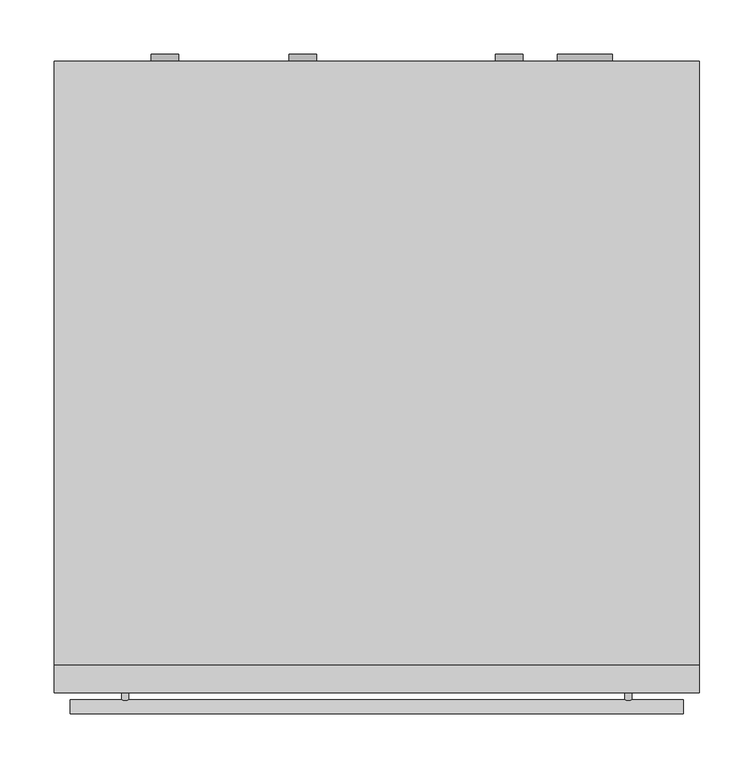
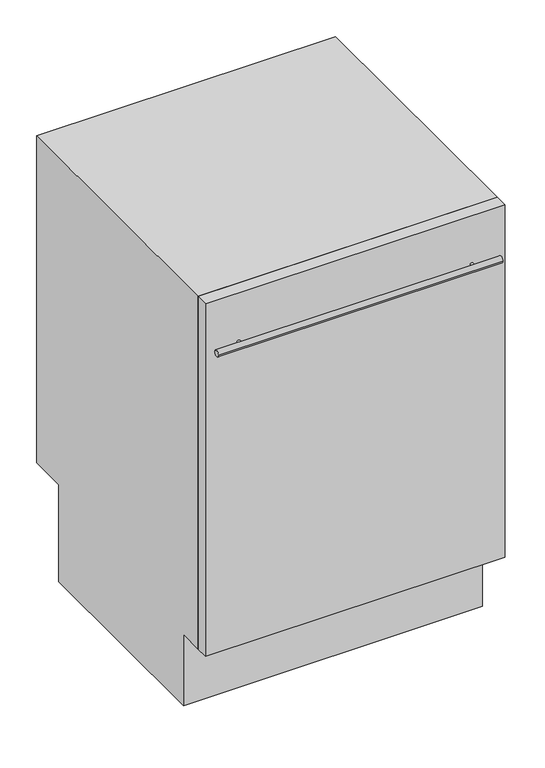
"""IFC4 building model written with IfcOpenShell, lengths in millimetres: proxy geometry, Dishwashers_GE-Monogram_ZBD9900RII : Dishwashers_GE-Monogram_ZBD9900RII."""

from ifc_helpers import new_model, si_unit, point, frame, frame_2d, origin, place, context, project, spatial, polyline, circle_curve, trimmed, segment, composite_curve, outline, extrude, source, transform, mapped, element, save


def specialty_equipment_35477451(model_context):
    return source(origin(), model_context, "Body", "SweptSolid", [
        extrude(outline(composite_curve([segment(trimmed(circle_curve(frame_2d((786.8961152, -231.5904925)), 3.175), [point((786.8961152, -234.7654925))], [point((786.8961152, -228.4154925))], False, "CARTESIAN"), True, "CONTINUOUS"), segment(trimmed(circle_curve(frame_2d((786.8961152, -231.5904925)), 3.175), [point((786.8961152, -228.4154925))], [point((786.8961152, -234.7654925))], False, "CARTESIAN"), True, "CONTINUOUS")], self_intersect=False)), frame((0.0, -307.975, 0.0), z_axis=(0.0, 1.0, 0.0), x_axis=(0.0, 0.0, 1.0)), (0.0, 0.0, 1.0), 12.7),
        extrude(outline(composite_curve([segment(trimmed(circle_curve(frame_2d((786.8961152, 231.5904925)), 3.175), [point((786.8961152, 228.4154925))], [point((786.8961152, 234.7654925))], False, "CARTESIAN"), True, "CONTINUOUS"), segment(trimmed(circle_curve(frame_2d((786.8961152, 231.5904925)), 3.175), [point((786.8961152, 234.7654925))], [point((786.8961152, 228.4154925))], False, "CARTESIAN"), True, "CONTINUOUS")], self_intersect=False)), frame((0.0, -307.975, 0.0), z_axis=(0.0, 1.0, 0.0), x_axis=(0.0, 0.0, 1.0)), (0.0, 0.0, 1.0), 12.7),
        extrude(outline(composite_curve([segment(trimmed(circle_curve(frame_2d((-307.975, 787.4)), 6.35), [point((-314.325, 787.4))], [point((-301.625, 787.4))], False, "CARTESIAN"), True, "CONTINUOUS"), segment(trimmed(circle_curve(frame_2d((-307.975, 787.4)), 6.35), [point((-301.625, 787.4))], [point((-314.325, 787.4))], False, "CARTESIAN"), True, "CONTINUOUS")], self_intersect=False)), frame((-282.3904925, 0.0, 0.0), z_axis=(1.0, 0.0, 0.0), x_axis=(0.0, 1.0, 0.0)), (0.0, 0.0, 1.0), 564.780985),
        extrude(outline(polyline([(296.8625, -269.875), (296.8625, -295.275), (-296.8625, -295.275), (-296.8625, -269.875), (296.8625, -269.875)])), frame((0.0, 0.0, 149.225), z_axis=(0.0, 0.0, 1.0), x_axis=(1.0, 0.0, 0.0)), (0.0, 0.0, 1.0), 739.775),
        extrude(outline(polyline([(209.55, 0.0), (-219.075, 0.0), (-219.075, 149.225), (-269.875, 149.225), (-269.875, 889.0), (285.75, 889.0), (285.75, 203.2), (209.55, 203.2), (209.55, 0.0)])), frame((-296.8625, 0.0, 0.0), z_axis=(1.0, 0.0, 0.0), x_axis=(0.0, 1.0, 0.0)), (0.0, 0.0, 1.0), 593.725),
        extrude(outline(composite_curve([segment(trimmed(circle_curve(frame_2d((141.5005288, 191.4753985)), 25.4), [point((141.5005288, 216.8753985))], [point((141.5005288, 166.0753985))], False, "CARTESIAN"), True, "CONTINUOUS"), segment(trimmed(circle_curve(frame_2d((141.5005288, 191.4753985)), 25.4), [point((141.5005288, 166.0753985))], [point((141.5005288, 216.8753985))], False, "CARTESIAN"), True, "CONTINUOUS")], self_intersect=False)), frame((0.0, 285.75, 0.0), z_axis=(0.0, 1.0, 0.0), x_axis=(0.0, 0.0, 1.0)), (0.0, 0.0, 1.0), 6.35),
        extrude(outline(composite_curve([segment(trimmed(circle_curve(frame_2d((292.1857454, -195.1522721)), 12.7), [point((292.1857454, -182.4522721))], [point((292.1857454, -207.8522721))], False, "CARTESIAN"), True, "CONTINUOUS"), segment(trimmed(circle_curve(frame_2d((292.1857454, -195.1522721)), 12.7), [point((292.1857454, -207.8522721))], [point((292.1857454, -182.4522721))], False, "CARTESIAN"), True, "CONTINUOUS")], self_intersect=False)), frame((0.0, 285.75, 0.0), z_axis=(0.0, 1.0, 0.0), x_axis=(0.0, 0.0, 1.0)), (0.0, 0.0, 1.0), 6.35),
        extrude(outline(composite_curve([segment(trimmed(circle_curve(frame_2d((314.6288473, -68.0887314)), 12.7), [point((314.6288473, -55.3887314))], [point((314.6288473, -80.7887314))], False, "CARTESIAN"), True, "CONTINUOUS"), segment(trimmed(circle_curve(frame_2d((314.6288473, -68.0887314)), 12.7), [point((314.6288473, -80.7887314))], [point((314.6288473, -55.3887314))], False, "CARTESIAN"), True, "CONTINUOUS")], self_intersect=False)), frame((0.0, 285.75, 0.0), z_axis=(0.0, 1.0, 0.0), x_axis=(0.0, 0.0, 1.0)), (0.0, 0.0, 1.0), 6.35),
        extrude(outline(composite_curve([segment(trimmed(circle_curve(frame_2d((278.7164133, 121.739524)), 12.7), [point((278.7164133, 134.439524))], [point((278.7164133, 109.039524))], False, "CARTESIAN"), True, "CONTINUOUS"), segment(trimmed(circle_curve(frame_2d((278.7164133, 121.739524)), 12.7), [point((278.7164133, 109.039524))], [point((278.7164133, 134.439524))], False, "CARTESIAN"), True, "CONTINUOUS")], self_intersect=False)), frame((0.0, 285.75, 0.0), z_axis=(0.0, 1.0, 0.0), x_axis=(0.0, 0.0, 1.0)), (0.0, 0.0, 1.0), 6.35),
    ])


if __name__ == "__main__":
    model = new_model("IFC4")
    model_context = context("Model", 3, world=origin())
    ifc_project = project(units=[si_unit("LENGTHUNIT", "METRE", prefix="MILLI")], contexts=[model_context])
    site = spatial("IfcSite", under=ifc_project)
    building = spatial("IfcBuilding", under=site)
    placement = place(None, origin())
    specialty_equipment_shape = specialty_equipment_35477451(model_context)
    element("IfcBuildingElementProxy", 1, Name="Dishwashers_GE-Monogram_ZBD9900RII : Dishwashers_GE-Monogram_ZBD9900RII", ObjectType="Dishwashers_GE-Monogram_ZBD9900RII : Dishwashers_GE-Monogram_ZBD9900RII", at=placement, inside=building, context=model_context, shape_type="MappedRepresentation", body=[
        mapped(specialty_equipment_shape, transform((0.0, 0.0, 0.0), x_axis=(1.0, 0.0, 0.0), y_axis=(0.0, 1.0, 0.0), z_axis=(0.0, 0.0, 1.0))),
    ])
    save(model, "model.ifc")

# Revit data of these elements
# Type "Dishwashers_GE-Monogram_ZBD9900RII : Dishwashers_GE-Monogram_ZBD9900RII"
#   COBie.Type.CreatedBy = "design@eagle.com"
#   COBie.Type.CreatedOn = "2016-10-27T05:31:12"
#   COBie.Type.Name = "Dishwashers_GE-Monogram_ZBD9900RII_Dishwashers_GE-Monogram_ZBD9900RII"
#   COBie.Type.Category = "23-45 30 11 11 : Residential Dishwashers"
#   COBie.Type.Description = "Dishwashers_GE-Monogram_ZBD9900RII_Dishwashers_GE-Monogram_ZBD9900RII"
#   COBie.Type.Manufacturer = "info@geappliances.com"
#   COBie.Type.ModelNumber = "As Specified in 11 30 00"
#   Wash Cycles = ""
#   URL = "http://www.geappliances.com/"
#   Test Data = "http://www.geappliances.com/service_and_support/search.htm"
#   Specification = "http://www.arcat.com/sdspecs/htm/11450gea.htm"
#   SpecWizard = "http://www.arcat.com/specwizard/11450gea/index.htm?mf=&coid=32703"
#   Send Message = "http://www.arcat.com/users.pl?action=UserEmail&company=GE%20Appliances&coid=32703&rep=114&fax=502-452-0620&mf="
#   Sales Information = "http://www.geappliances.com/buy/"
#   Revision = "R1_02-2011"
#   Product Properties = "http://www.arcat.com/bim/bim_info.pl?fn=GEAppliances"
#   Product Data = "http://www.arcat.com/arcatcos/cos32/arc32703.html"
#   Model = "As Specified in 11 30 00"
#   Manufacturer Website = "http://www.geappliances.com/"
#   Manufacturer Phone - Toll Free = "800-626-2000"
#   Manufacturer Phone = "502-452-3346"
#   Manufacturer Fax = "502-452-0620"
#   Manufacturer Address = "Appliance Park AP4-109, Louisville, KY 40225"
#   Manufacturer = "info@geappliances.com"
#   Keynote = "11 30 00"
#   Installation-Fabrication = "http://www.geappliances.com/service_and_support/literature/"
#   Installation Phase = ""
#   Green Building-LEED = "http://www.geappliances.com/energy-star-appliances/"
#   ENERGYSTAR Qualified = ""
#   Drawn By = "Sumex Design, Inc. / Robert S. Weygant, CSI, CDT, SCIP"
#   Description = "Residential Appliance as Specified in 11 30 00"
#   Copyright = "©Arcat Inc."
#   Construction Details = "http://www.geappliances.com/design_center/"
#   Building Codes = "http://www.geappliances.com/service_and_support/search.htm"
#   Assembly Code = "E1090400"
#   COBie.Type.ReplacementCost = 0
#   offset [instance default] = 0' - 0"
#   Voltage_MEP = 120 V
#   Unit Width = 1' - 11 3/8"
#   Unit Height = 2' - 11"
#   Unit Depth = 1' - 10 7/8"
#   MEP Apparent Power = 60 VA
#   MEP Amperage = 0.5 A
#   HWRad = 0' - 0 1/4"
#   GasRad = 0' - 0 1/4"
#   DrainRad = 0' - 0 5/8"
#   Connection Dia HW = 0' - 0 1/2"
#   Connection Dia Gas = 0' - 0 1/2"
#   Connection Dia DWV = 0' - 1 1/4"
#   Connection Dia CW = 0' - 0 1/2"
#   CWRad = 0' - 0 1/4"
#   COBie.Type = yes
#   Warranty Duration (Years) = 0
#   Maintenance Schedule (Months) = 0
#   Expected Lifespan (Years) = 0
#   ADA Compliant = yes
#   Handle Finish = none
#   Exterior Finish = ARCAT - Finish - Stainless steel
# Element 1 (IfcBuildingElementProxy, "Dishwashers_GE-Monogram_ZBD9900RII : Dishwashers_GE-Monogram_ZBD9900RII")
#   Materials on its faces: "ARCAT - Finish - Stainless steel", "Sanitary", "Hot", "Cold", "Connector"
# Materials
#   "ARCAT - Finish - Stainless steel": class "Unassigned", colour RGB 244 244 244, transparency 0, Keynote = "09910", Model = "Generic", Manufacturer = "Generic", Description = "Paints"
#   "Sanitary": class "Miscellaneous", colour RGB 0 255 0, transparency 0
#   "Hot": class "Miscellaneous", colour RGB 255 0 0, transparency 0
#   "Cold": class "Miscellaneous", colour RGB 0 0 255, transparency 0
#   "Connector": class "Miscellaneous", colour RGB 255 255 0, transparency 0
